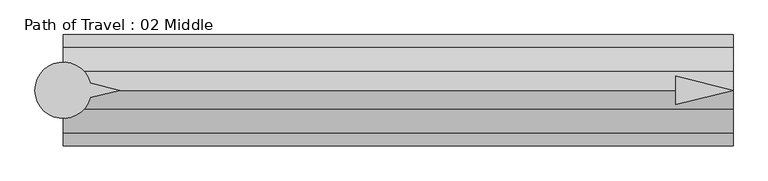
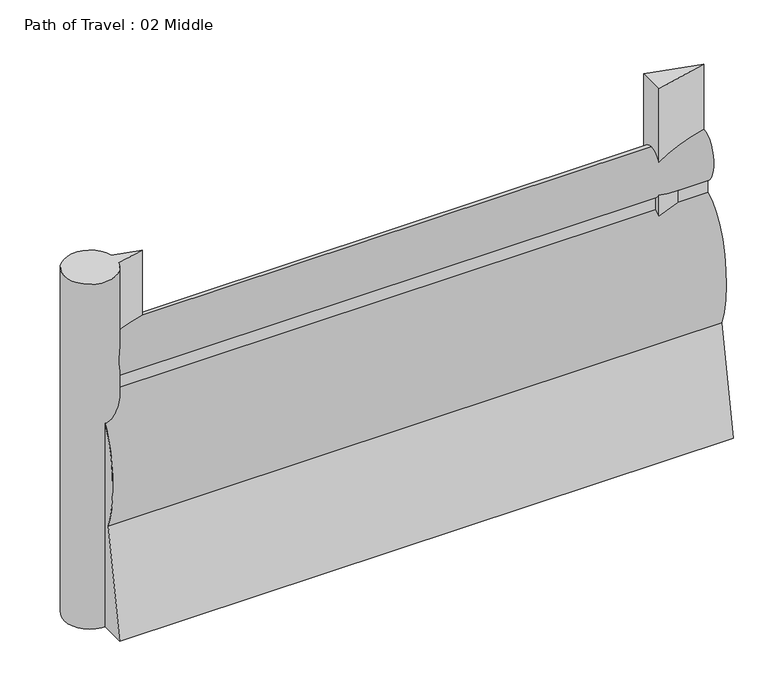
"""IFC4 building model written with IfcOpenShell, lengths in millimetres: proxy geometry, Path of Travel : 02 Middle."""

from ifc_helpers import new_model, si_unit, point, frame, frame_2d, origin, origin_with_axes, place, context, project, spatial, polyline, circle_curve, ellipse_curve, trimmed, segment, composite_curve, outline, extrude, source, transform, mapped, element, save
from ifc_brep_helpers import plane_surface, extruded_surface, advanced_brep


def path_of_travel_02_middle_e7a0fddd(model_context):
    return source(origin(), model_context, "Body", "SolidModel", [
        advanced_brep(
        [(227.5554837, 0.0, 1727.2), (227.5554837, 42.9018657, 1436.6534209), (227.5554837, 42.9018657, 1363.4763406), (227.5554837, 184.1186263, 643.4144547), (227.5554837, 297.5699544, 0.0), (227.5554837, 145.6574193, 0.0), (227.5554837, 0.0, 584.2), (227.5554837, -145.6574193, 0.0), (227.5554837, -297.5699544, 0.0), (227.5554837, -184.1186263, 643.4144547), (227.5554837, -42.9018657, 1363.4763406), (227.5554837, -42.9018657, 1436.6534209), (3811.0623095, 0.0, 1727.2), (3811.0623095, -42.9018657, 1436.6534209), (3811.0623095, -42.9018657, 1363.4763406), (3811.0623095, -184.1186263, 643.4144547), (3811.0623095, -297.5699544, 0.0), (3811.0623095, -145.6574193, 0.0), (3811.0623095, 0.0, 584.2), (3811.0623095, 145.6574193, 0.0), (3811.0623095, 297.5699544, 0.0), (3811.0623095, 184.1186263, 643.4144547), (3811.0623095, 42.9018657, 1363.4763406), (3811.0623095, 42.9018657, 1436.6534209)],
        [
            (0, 1, ellipse_curve(frame((227.5554837, 0.0, 1574.8), z_axis=(-1.0, 0.0, 0.0), x_axis=(0.0, 0.0, 1.0)), 152.4, 101.6)),
            (1, 2),
            (2, 3, ellipse_curve(frame((227.5554837, 0.0, 914.4), z_axis=(-1.0, 0.0, 0.0), x_axis=(0.0, 0.0, -1.0)), 457.2, 228.6)),
            (3, 4),
            (4, 5),
            (5, 6),
            (6, 7),
            (7, 8),
            (8, 9),
            (9, 10, ellipse_curve(frame((227.5554837, 0.0, 914.4), z_axis=(-1.0, 0.0, 0.0), x_axis=(0.0, 0.0, -1.0)), 457.2, 228.6)),
            (10, 11),
            (11, 0, ellipse_curve(frame((227.5554837, 0.0, 1574.8), z_axis=(-1.0, 0.0, 0.0), x_axis=(0.0, 0.0, 1.0)), 152.4, 101.6)),
            (12, 13, ellipse_curve(frame((3811.0623095, 0.0, 1574.8), z_axis=(1.0, 0.0, 0.0), x_axis=(0.0, 0.0, 1.0)), 152.4, 101.6)),
            (13, 14),
            (14, 15, ellipse_curve(frame((3811.0623095, 0.0, 914.4), z_axis=(1.0, 0.0, 0.0), x_axis=(0.0, 0.0, -1.0)), 457.2, 228.6)),
            (15, 16),
            (16, 17),
            (17, 18),
            (18, 19),
            (19, 20),
            (20, 21),
            (21, 22, ellipse_curve(frame((3811.0623095, 0.0, 914.4), z_axis=(1.0, 0.0, 0.0), x_axis=(0.0, 0.0, -1.0)), 457.2, 228.6)),
            (22, 23),
            (23, 12, ellipse_curve(frame((3811.0623095, 0.0, 1574.8), z_axis=(1.0, 0.0, 0.0), x_axis=(0.0, 0.0, 1.0)), 152.4, 101.6)),
            (0, 12),
            (23, 1),
            (22, 2),
            (21, 3),
            (20, 4),
            (19, 5),
            (18, 6),
            (17, 7),
            (16, 8),
            (15, 9),
            (14, 10),
            (13, 11),
        ],
        [
            plane_surface(frame((227.5554837, 0.0, 0.0), z_axis=(-1.0, 0.0, 0.0), x_axis=(0.0, 0.0, 1.0))),
            plane_surface(frame((3811.0623095, 0.0, 0.0), z_axis=(1.0, 0.0, 0.0), x_axis=(0.0, 0.0, 1.0))),
            extruded_surface(trimmed(ellipse_curve(frame((3811.0623095, 0.0, 1574.8), z_axis=(-1.0, 0.0, 0.0), x_axis=(0.0, 0.0, 1.0)), 152.4, 101.6), [point((3811.0623095, 0.0, 1727.2))], [point((3811.0623095, 42.9018657, 1436.6534209))], True, "CARTESIAN"), (-3583.5068258, 0.0, 0.0), 3583.5068258),
            plane_surface(frame((227.5554837, 42.9018657, 1436.6534209), z_axis=(0.0, 1.0, 0.0), x_axis=(1.0, 0.0, 0.0))),
            extruded_surface(trimmed(ellipse_curve(frame((3811.0623095, 0.0, 914.4), z_axis=(-1.0, 0.0, 0.0), x_axis=(0.0, 0.0, -1.0)), 457.2, 228.6), [point((3811.0623095, 42.9018657, 1363.4763406))], [point((3811.0623095, 184.1186263, 643.4144547))], True, "CARTESIAN"), (-3583.5068258, 0.0, 0.0), 3583.5068258),
            plane_surface(frame((227.5554837, 184.1186263, 643.4144547), z_axis=(0.0, 0.9848077530122078, 0.1736481776669322), x_axis=(1.0, 0.0, 0.0))),
            plane_surface(frame((227.5554837, 297.5699544, 0.0), z_axis=(0.0, 0.0, -1.0), x_axis=(1.0, 0.0, 0.0))),
            plane_surface(frame((227.5554837, 145.6574193, 0.0), z_axis=(0.0, -0.9702957262760199, -0.2419218955995739), x_axis=(1.0, 0.0, 0.0))),
            plane_surface(frame((227.5554837, 0.0, 584.2), z_axis=(0.0, 0.9702957262759961, -0.24192189559966923), x_axis=(1.0, 0.0, 0.0))),
            plane_surface(frame((227.5554837, -145.6574193, 0.0), z_axis=(0.0, 0.0, -1.0), x_axis=(1.0, 0.0, 0.0))),
            plane_surface(frame((227.5554837, -297.5699544, 0.0), z_axis=(0.0, -0.984807753012208, 0.17364817766693066), x_axis=(1.0, 0.0, 0.0))),
            extruded_surface(trimmed(ellipse_curve(frame((3811.0623095, 0.0, 914.4), z_axis=(-1.0, 0.0, 0.0), x_axis=(0.0, 0.0, -1.0)), 457.2, 228.6), [point((3811.0623095, -184.1186263, 643.4144547))], [point((3811.0623095, -42.9018657, 1363.4763406))], True, "CARTESIAN"), (-3583.5068258, 0.0, 0.0), 3583.5068258),
            plane_surface(frame((227.5554837, -42.9018657, 1363.4763406), z_axis=(0.0, -1.0, 0.0), x_axis=(1.0, 0.0, 0.0))),
            extruded_surface(trimmed(ellipse_curve(frame((3811.0623095, 0.0, 1574.8), z_axis=(-1.0, 0.0, 0.0), x_axis=(0.0, 0.0, 1.0)), 152.4, 101.6), [point((3811.0623095, -42.9018657, 1436.6534209))], [point((3811.0623095, 0.0, 1727.2))], True, "CARTESIAN"), (-3583.5068258, 0.0, 0.0), 3583.5068258),
        ],
        [
            (0, [[1, 2, 3, 4, 5, 6, 7, 8, 9, 10, 11, 12]]),
            (1, [[13, 14, 15, 16, 17, 18, 19, 20, 21, 22, 23, 24]]),
            (2, [[-1, 25, -24, 26]]),
            (3, [[-2, -26, -23, 27]]),
            (4, [[-3, -27, -22, 28]]),
            (5, [[-4, -28, -21, 29]]),
            (6, [[-5, -29, -20, 30]]),
            (7, [[-6, -30, -19, 31]]),
            (8, [[-7, -31, -18, 32]]),
            (9, [[-8, -32, -17, 33]]),
            (10, [[-9, -33, -16, 34]]),
            (11, [[-10, -34, -15, 35]]),
            (12, [[-11, -35, -14, 36]]),
            (13, [[-12, -36, -13, -25]]),
        ],
    ),
        extrude(outline(polyline([(3505.057163, 76.2006338), (3811.0623095, 0.0), (3505.057163, -76.2006338), (3505.057163, 76.2006338)])), origin_with_axes(), (0.0, 0.0, 1.0), 2129.5973753),
        extrude(outline(composite_curve([segment(polyline([(372.7837828, 39.4440225), (531.182385, 0.0), (372.7837828, -39.4440225)]), True, "CONTINUOUS"), segment(trimmed(circle_curve(frame_2d((227.2200886, 0.0)), 150.8131956), [point((372.7837828, -39.4440225))], [point((372.7837828, 39.4440225))], False, "CARTESIAN"), True, "CONTINUOUS")], self_intersect=False)), origin_with_axes(), (0.0, 0.0, 1.0), 2129.5973753),
    ])


if __name__ == "__main__":
    model = new_model("IFC4")
    model_context = context("Model", 3, world=origin())
    ifc_project = project(units=[si_unit("LENGTHUNIT", "METRE", prefix="MILLI")], contexts=[model_context])
    site = spatial("IfcSite", under=ifc_project)
    building = spatial("IfcBuilding", under=site)
    placement = place(None, origin())
    path_of_travel_02_middle_shape = path_of_travel_02_middle_e7a0fddd(model_context)
    element("IfcBuildingElementProxy", 1, Name="Path of Travel : 02 Middle", ObjectType="Path of Travel : 02 Middle", at=placement, inside=building, context=model_context, shape_type="MappedRepresentation", body=[
        mapped(path_of_travel_02_middle_shape, transform((0.0, 0.0, 0.0), x_axis=(1.0, 0.0, 0.0), y_axis=(0.0, 1.0, 0.0), z_axis=(0.0, 0.0, 1.0))),
    ])
    save(model, "model.ifc")

# Revit data of these elements
# Type "Path of Travel : 02 Middle"
#   Path of Egress [instance default] = 4' - 0"
#   built-in parameter 1001306 [instance default] = 4 (stored number, unit not read)
#   Dot at Start = no
#   Arrow in Middle = yes
#   Arrow at End = no
#   Egress Path = none
# Element 1 (IfcBuildingElementProxy, "Path of Travel : 02 Middle")
#   Path of Egress = 11' - 9.08295"
#   built-in parameter 1001306 = 11.7569 (stored number, unit not read)
